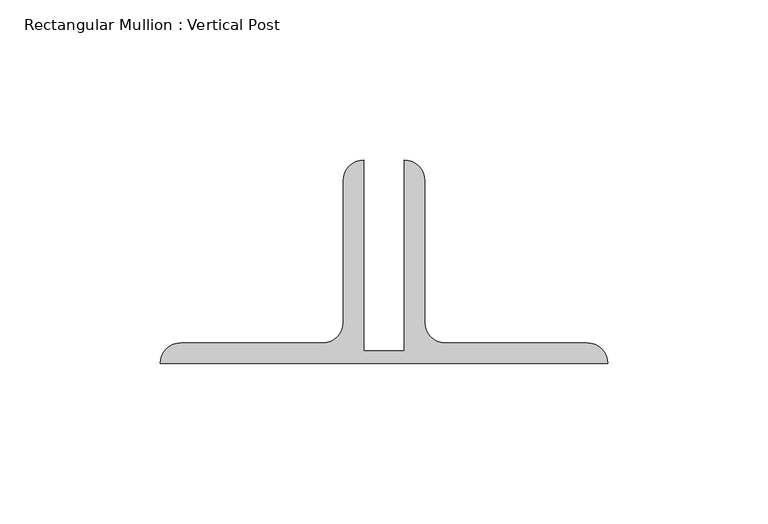
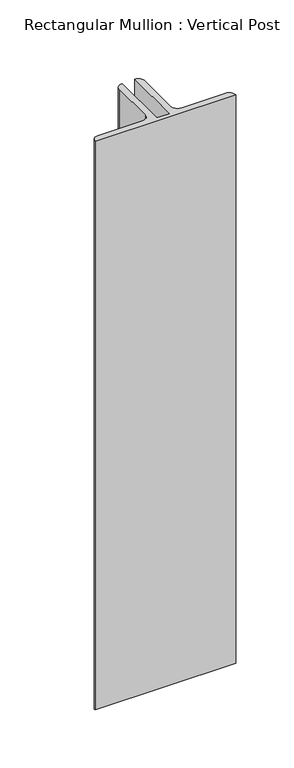
"""IFC4 building model written with IfcOpenShell, lengths in millimetres: member geometry, Rectangular Mullion : Vertical Post."""

import ifcopenshell
import ifcopenshell.guid

model = None  # the IFC model being written
_history = None  # IfcOwnerHistory: only IFC2X3 demands one
_inside = {}  # id of a spatial element -> (the spatial element, [elements in it])
_under = {}  # id of a project, library or spatial element -> (it, [spatial elements below it])
_declared = {}  # id of a project -> (the project, [libraries it declares])
_typed = {}  # id of a type object -> (the type object, [elements of that type])
_made_of = {}  # id of a material, layer set ... -> (it, [elements and type objects made of it])


def new_model(schema):
    """Start an empty IFC model of exactly this schema.

    Asked for "IFC4X3", IfcOpenShell would pick the latest addendum, in which some entities
    have other attributes; the version numbers below select the first issue.
    IFC2X3 requires an IfcOwnerHistory on every rooted entity: one is made here for all.
    """
    global model, _history
    if schema == "IFC4X3":
        model = ifcopenshell.file(schema_version=(4, 3, 0, 0))
    else:
        model = ifcopenshell.file(schema=schema)
    _inside.clear()
    _under.clear()
    _declared.clear()
    _typed.clear()
    _made_of.clear()
    _history = None
    if model.schema == "IFC2X3":
        org = make("IfcOrganization", Name="unknown")
        user = make(
            "IfcPersonAndOrganization",
            ThePerson=make("IfcPerson", FamilyName="unknown"),
            TheOrganization=org,
        )
        app = make(
            "IfcApplication",
            ApplicationDeveloper=org,
            Version="unknown",
            ApplicationFullName="unknown",
            ApplicationIdentifier="unknown",
        )
        _history = make(
            "IfcOwnerHistory",
            OwningUser=user,
            OwningApplication=app,
            ChangeAction="ADDED",
            CreationDate=0,
        )
    return model


def make(cls, **values):
    """One entity of the class cls with the attributes given. An attribute that is None is left unset."""
    return model.create_entity(
        cls, **{name: value for name, value in values.items() if value is not None}
    )


def rooted(cls, **values):
    """An entity with a GlobalId (a new one), such as an element, a storey or a relation."""
    return make(cls, GlobalId=ifcopenshell.guid.new(), OwnerHistory=_history, **values)


def si_unit(unit_type, name, prefix=None):
    """IfcSIUnit, for example si_unit("LENGTHUNIT", "METRE", prefix="MILLI")."""
    return make("IfcSIUnit", UnitType=unit_type, Prefix=prefix, Name=name)


def assignment(units):
    """IfcUnitAssignment: the units of a project."""
    return None if units is None else make("IfcUnitAssignment", Units=units)


def point(xyz):
    """IfcCartesianPoint."""
    return None if xyz is None else make("IfcCartesianPoint", Coordinates=xyz)


def direction(xyz):
    """IfcDirection."""
    return None if xyz is None else make("IfcDirection", DirectionRatios=xyz)


def frame(location, z_axis=None, x_axis=None):
    """IfcAxis2Placement3D, a coordinate frame: its origin and axes. An axis left out is left unset."""
    return make(
        "IfcAxis2Placement3D",
        Location=point(location),
        Axis=direction(z_axis),
        RefDirection=direction(x_axis),
    )


def frame_2d(location, x_axis=None):
    """IfcAxis2Placement2D, a coordinate frame in the plane: its origin and x axis."""
    return make(
        "IfcAxis2Placement2D", Location=point(location), RefDirection=direction(x_axis)
    )


def origin():
    """The frame at (0, 0, 0) with its axes left unset."""
    return frame((0.0, 0.0, 0.0))


def place(relative_to, where):
    """IfcLocalPlacement: puts the frame where relative to a parent placement (None: the world)."""
    return make(
        "IfcLocalPlacement", PlacementRelTo=relative_to, RelativePlacement=where
    )


def context(
    kind, dimensions, precision=None, world=None, true_north=None, identifier=None
):
    """IfcGeometricRepresentationContext, for example the 3D "Model" context."""
    return make(
        "IfcGeometricRepresentationContext",
        ContextIdentifier=identifier,
        ContextType=kind,
        CoordinateSpaceDimension=dimensions,
        Precision=precision,
        WorldCoordinateSystem=world,
        TrueNorth=true_north,
    )


def project(units=None, contexts=None):
    """IfcProject with its units and contexts."""
    return rooted(
        "IfcProject",
        Name="project",
        RepresentationContexts=contexts,
        UnitsInContext=assignment(units),
    )


def spatial(cls, under=None, at=None, **own):
    """A site, building, storey or space (cls), placed at a placement, below another one or the project."""
    s = rooted(cls, ObjectPlacement=at, **own)
    if under is not None:
        _under.setdefault(under.id(), (under, []))[1].append(s)
    return s


def polyline(points):
    """IfcPolyline through the points."""
    return make("IfcPolyline", Points=[point(p) for p in points])


def circle_curve(where, radius):
    """IfcCircle in the frame where."""
    return make("IfcCircle", Position=where, Radius=radius)


def trimmed(basis, trim1, trim2, sense, master):
    """IfcTrimmedCurve: the piece of a basis curve between two trims."""
    return make(
        "IfcTrimmedCurve",
        BasisCurve=basis,
        Trim1=trim1,
        Trim2=trim2,
        SenseAgreement=sense,
        MasterRepresentation=master,
    )


def segment(curve, same_sense, transition):
    """IfcCompositeCurveSegment."""
    return make(
        "IfcCompositeCurveSegment",
        Transition=transition,
        SameSense=same_sense,
        ParentCurve=curve,
    )


def composite_curve(segments, self_intersect=None):
    """IfcCompositeCurve: segments joined end to end."""
    return make("IfcCompositeCurve", Segments=segments, SelfIntersect=self_intersect)


def outline(outer, holes=None, kind="AREA"):
    """IfcArbitraryClosedProfileDef: a profile drawn as a closed curve; with holes, ...WithVoids."""
    if holes is None:
        return make("IfcArbitraryClosedProfileDef", ProfileType=kind, OuterCurve=outer)
    return make(
        "IfcArbitraryProfileDefWithVoids",
        ProfileType=kind,
        OuterCurve=outer,
        InnerCurves=holes,
    )


def extrude(swept, where, along, depth):
    """IfcExtrudedAreaSolid: the profile swept, set in the frame where, extruded along a direction by depth."""
    return make(
        "IfcExtrudedAreaSolid",
        SweptArea=swept,
        Position=where,
        ExtrudedDirection=direction(along),
        Depth=depth,
    )


def shape(context_of_items, identifier, shape_type, items):
    """IfcShapeRepresentation: the items that make up one representation, for example the "Body"."""
    return make(
        "IfcShapeRepresentation",
        ContextOfItems=context_of_items,
        RepresentationIdentifier=identifier,
        RepresentationType=shape_type,
        Items=items,
    )


def source(mapping_origin, context_of_items, identifier, shape_type, items):
    """IfcRepresentationMap: a shape defined once, which mapped items show again and again."""
    return make(
        "IfcRepresentationMap",
        MappingOrigin=mapping_origin,
        MappedRepresentation=shape(context_of_items, identifier, shape_type, items),
    )


def transform(
    local_origin,
    x_axis=None,
    y_axis=None,
    z_axis=None,
    scale=None,
    scale2=None,
    scale3=None,
    uniform=True,
):
    """IfcCartesianTransformationOperator3D, or its non-uniform kind. x_axis, y_axis, z_axis: its Axis1, 2, 3."""
    if uniform:
        return make(
            "IfcCartesianTransformationOperator3D",
            Axis1=direction(x_axis),
            Axis2=direction(y_axis),
            LocalOrigin=point(local_origin),
            Scale=scale,
            Axis3=direction(z_axis),
        )
    return make(
        "IfcCartesianTransformationOperator3DnonUniform",
        Axis1=direction(x_axis),
        Axis2=direction(y_axis),
        LocalOrigin=point(local_origin),
        Scale=scale,
        Axis3=direction(z_axis),
        Scale2=scale2,
        Scale3=scale3,
    )


def mapped(mapping_source, mapping_target):
    """IfcMappedItem: shows the shape of a source again, moved by a transform."""
    return make(
        "IfcMappedItem", MappingSource=mapping_source, MappingTarget=mapping_target
    )


def made_of(thing, what):
    """Note that an element or type object is made of a material, layer set ...; save() writes the relation."""
    if what is not None:
        _made_of.setdefault(what.id(), (what, []))[1].append(thing)
    return thing


def element(
    cls,
    number,
    at=None,
    inside=None,
    cuts=None,
    type_object=None,
    material=None,
    context=None,
    identifier="Body",
    shape_type=None,
    held_by="IfcProductDefinitionShape",
    body=None,
    shapes=None,
    **own,
):
    """One element of the class cls, such as IfcWall. Its Tag is "e" and its number.

    at: its placement. inside: the storey or other place that contains it. cuts: it is an
    opening in that element (IfcRelVoidsElement). A single representation is given by context,
    identifier, shape_type and body (its items); several are given by shapes. held_by: the class
    of the entity that holds the representations. save() writes the other relations.
    """
    e = rooted(cls, Tag="e%d" % number, ObjectPlacement=at, **own)
    if body is not None:
        shapes = [shape(context, identifier, shape_type, body)]
    if shapes is not None:
        e.Representation = make(held_by, Representations=shapes)
    if inside is not None:
        _inside.setdefault(inside.id(), (inside, []))[1].append(e)
    if cuts is not None:
        rooted(
            "IfcRelVoidsElement", RelatingBuildingElement=cuts, RelatedOpeningElement=e
        )
    if type_object is not None:
        _typed.setdefault(type_object.id(), (type_object, []))[1].append(e)
    return made_of(e, material)


def aggregate(whole, parts):
    """IfcRelAggregates: a whole, such as a stair, and the parts it consists of."""
    return rooted("IfcRelAggregates", RelatingObject=whole, RelatedObjects=parts)


def save(model, path):
    """Write the relations noted so far, then the file.

    IfcRelAggregates (storeys below a building ...), IfcRelContainedInSpatialStructure (elements
    in a storey), IfcRelDefinesByType, IfcRelAssociatesMaterial and IfcRelDeclares: one each for
    every whole, place, type object, material and project.
    """
    for whole, parts in _under.values():
        aggregate(whole, parts)
    for where, things in _inside.values():
        rooted(
            "IfcRelContainedInSpatialStructure",
            RelatedElements=things,
            RelatingStructure=where,
        )
    for kind, things in _typed.values():
        rooted("IfcRelDefinesByType", RelatedObjects=things, RelatingType=kind)
    for what, things in _made_of.values():
        rooted("IfcRelAssociatesMaterial", RelatedObjects=things, RelatingMaterial=what)
    for by, libraries in _declared.values():
        rooted("IfcRelDeclares", RelatingContext=by, RelatedDefinitions=libraries)
    model.write(path)


def rectangular_mullion_vertical_post_30249c29(model_context):
    return source(origin(), model_context, "Body", "SweptSolid", [
        extrude(outline(composite_curve([segment(polyline([(-63.5, 22.9145205), (-63.5, 82.55)]), True, "CONTINUOUS"), segment(trimmed(circle_curve(frame_2d((-63.5, 76.2)), 6.35), [point((-63.5, 82.55))], [point((-57.15, 76.2))], False, "CARTESIAN"), True, "CONTINUOUS"), segment(polyline([(-57.15, 76.2), (-57.15, 31.75)]), True, "CONTINUOUS"), segment(trimmed(circle_curve(frame_2d((-50.8, 31.75)), 6.35), [point((-57.15, 31.75))], [point((-50.8, 25.4))], True, "CARTESIAN"), True, "CONTINUOUS"), segment(polyline([(-50.8, 25.4), (-6.35, 25.4)]), True, "CONTINUOUS"), segment(trimmed(circle_curve(frame_2d((-6.35, 19.05)), 6.35), [point((-6.35, 25.4))], [point((0.0, 19.05))], False, "CARTESIAN"), True, "CONTINUOUS"), segment(polyline([(0.0, 19.05), (-139.7, 19.05)]), True, "CONTINUOUS"), segment(trimmed(circle_curve(frame_2d((-133.35, 19.05)), 6.35), [point((-139.7, 19.05))], [point((-133.35, 25.4))], False, "CARTESIAN"), True, "CONTINUOUS"), segment(polyline([(-133.35, 25.4), (-88.9, 25.4)]), True, "CONTINUOUS"), segment(trimmed(circle_curve(frame_2d((-88.9, 31.75)), 6.35), [point((-88.9, 25.4))], [point((-82.55, 31.75))], True, "CARTESIAN"), True, "CONTINUOUS"), segment(polyline([(-82.55, 31.75), (-82.55, 76.2)]), True, "CONTINUOUS"), segment(trimmed(circle_curve(frame_2d((-76.2, 76.2)), 6.35), [point((-82.55, 76.2))], [point((-76.2, 82.55))], False, "CARTESIAN"), True, "CONTINUOUS"), segment(polyline([(-76.2, 82.55), (-76.2, 22.9145205), (-63.5, 22.9145205)]), True, "CONTINUOUS")], self_intersect=False)), frame((0.0, 0.0, -596.9), z_axis=(0.0, 0.0, 1.0), x_axis=(1.0, 0.0, 0.0)), (0.0, 0.0, 1.0), 596.9),
    ])


if __name__ == "__main__":
    model = new_model("IFC4")
    model_context = context("Model", 3, world=origin())
    ifc_project = project(units=[si_unit("LENGTHUNIT", "METRE", prefix="MILLI")], contexts=[model_context])
    site = spatial("IfcSite", under=ifc_project)
    building = spatial("IfcBuilding", under=site)
    placement = place(None, origin())
    rectangular_mullion_vertical_post_shape = rectangular_mullion_vertical_post_30249c29(model_context)
    element("IfcMember", 1, ObjectType="Rectangular Mullion : Vertical Post", at=placement, inside=building, context=model_context, shape_type="MappedRepresentation", body=[
        mapped(rectangular_mullion_vertical_post_shape, transform((0.0, 0.0, 0.0), x_axis=(1.0, 0.0, 0.0), y_axis=(0.0, 1.0, 0.0), z_axis=(0.0, 0.0, 1.0))),
    ])
    save(model, "model.ifc")

# Revit data of these elements
# Type "Rectangular Mullion : Vertical Post"
#   built-in parameter 1007351 = -0.0625 (stored number, unit not read)
#   built-in parameter 1007322 = 0.0126789 (stored number, unit not read)
#   built-in parameter 1007321 = 0.229167 (stored number, unit not read)
#   built-in parameter 1007320 = 0.229167 (stored number, unit not read)
# Element 1 (IfcMember, "Rectangular Mullion : Vertical Post")
#   Materials on its faces: "GATE POST: (2) BACK/BACK GALVANIZED ANGLES"
# Materials
#   "GATE POST: (2) BACK/BACK GALVANIZED ANGLES": class "Unassigned", colour RGB 211 211 211, transparency 0, Cost = 0
